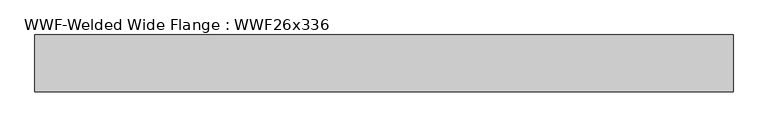
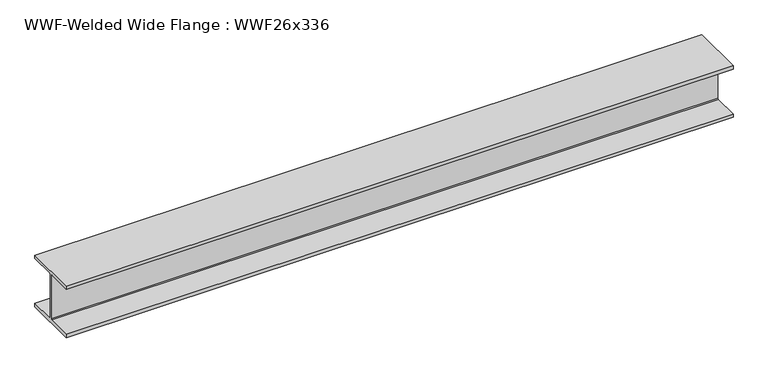
"""IFC4 building model written with IfcOpenShell, lengths in millimetres: beam geometry, WWF-Welded Wide Flange : WWF26x336."""

from ifc_helpers import new_model, si_unit, frame, origin, place, context, project, spatial, polyline, outline, extrude, source, transform, mapped, element, save


def wwf_welded_wide_flange_wwf26x336_ba16e7c2(model_context):
    return source(origin(), model_context, "Body", "SweptSolid", [
        extrude(outline(polyline([(324.993, -284.988), (324.993, -324.993), (-324.993, -324.993), (-324.993, -284.988), (-20.6375, -284.988), (-9.9949, -274.3454), (-9.9949, 274.3454), (-20.6375, 284.988), (-324.993, 284.988), (-324.993, 324.993), (324.993, 324.993), (324.993, 284.988), (20.6375, 284.988), (9.9949, 274.3454), (9.9949, -274.3454), (20.6375, -284.988), (324.993, -284.988)])), frame((-4064.2265761, 0.0, 0.0), z_axis=(1.0, 0.0, 0.0), x_axis=(0.0, 1.0, 0.0)), (0.0, 0.0, 1.0), 7999.1142873),
    ])


if __name__ == "__main__":
    model = new_model("IFC4")
    model_context = context("Model", 3, world=origin())
    ifc_project = project(units=[si_unit("LENGTHUNIT", "METRE", prefix="MILLI")], contexts=[model_context])
    site = spatial("IfcSite", under=ifc_project)
    building = spatial("IfcBuilding", under=site)
    placement = place(None, origin())
    wwf_welded_wide_flange_wwf26x336_shape = wwf_welded_wide_flange_wwf26x336_ba16e7c2(model_context)
    element("IfcBeam", 1, ObjectType="WWF-Welded Wide Flange : WWF26x336", at=placement, inside=building, context=model_context, shape_type="MappedRepresentation", body=[
        mapped(wwf_welded_wide_flange_wwf26x336_shape, transform((0.0, 0.0, 0.0), x_axis=(1.0, 0.0, 0.0), y_axis=(0.0, 1.0, 0.0), z_axis=(0.0, 0.0, 1.0))),
    ])
    save(model, "model.ifc")

# Revit data of these elements
# Type "WWF-Welded Wide Flange : WWF26x336"
#   Assembly Code = "B10"
#   Nominal d = "12"
#   W = 336
#   Length [instance default] = 1524 mm
#   bf = 649.986 mm
#   d = 649.986 mm
#   k = 20.638 mm
#   tf = 40.005 mm
#   tw = 19.99 mm
#   A = 0.0635483 m²
#   Structural Material [instance default] = Steel ASTM A572
# Element 1 (IfcBeam, "WWF-Welded Wide Flange : WWF26x336")
#   Structural Material = Metal - Steel 43-275
#   Materials on its faces: "Metal - Steel 43-275"
# Materials
#   "Steel ASTM A572": class "Metal", colour RGB 247 247 247, transparency 0, Description = "Structural steel, high strength low alloy, ASTM - A572 - 50", Cost = 0
#   "Metal - Steel 43-275": class "Metal", colour RGB 247 247 247, transparency 0, Cost = 0
